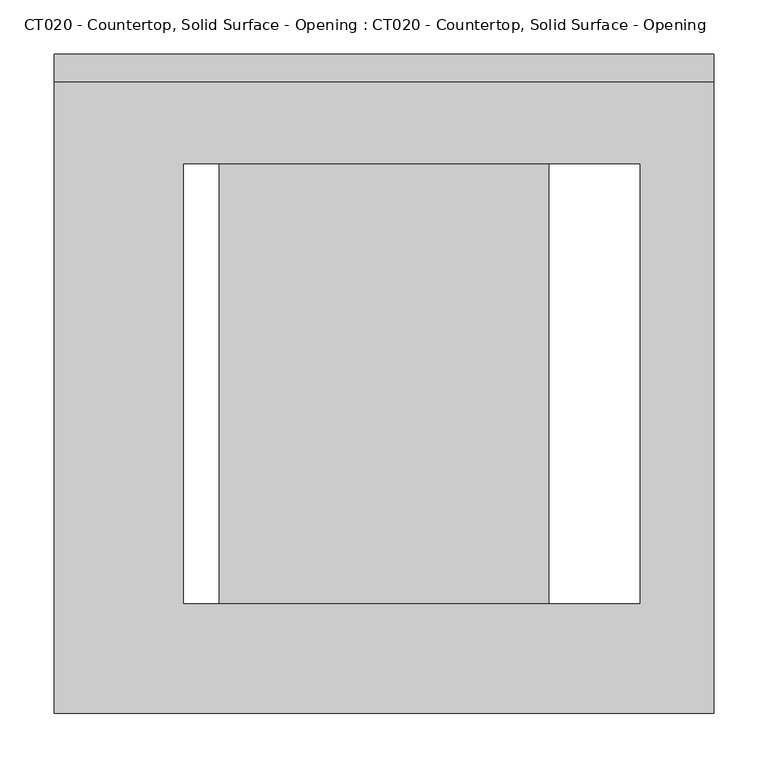
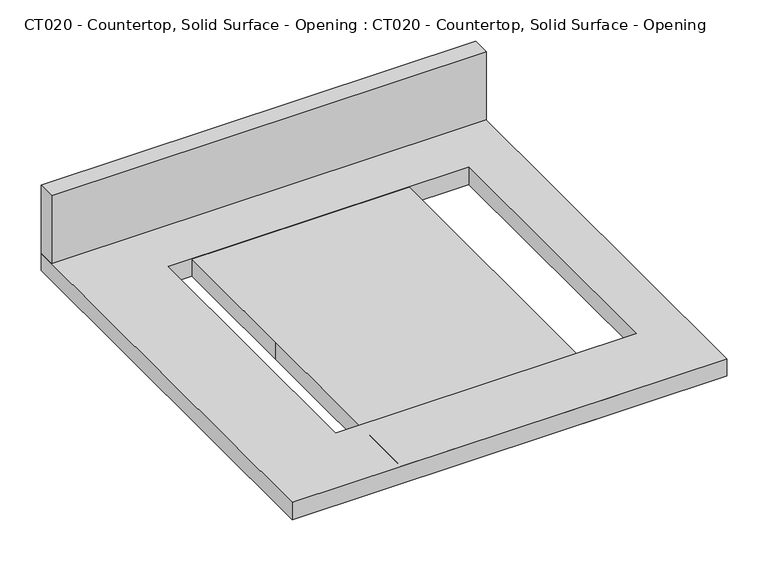
"""IFC4 building model written with IfcOpenShell, lengths in millimetres: proxy geometry, CT020 - Countertop, Solid Surface - Opening : CT020 - Countertop, Solid Surface - Opening."""

from ifc_helpers import new_model, si_unit, frame, origin, origin_with_axes, place, context, project, spatial, polyline, outline, extrude, source, transform, mapped, element, save


def ct020_countertop_solid_surface_opening_ct020_countertop_b7659a89(model_context):
    return source(origin(), model_context, "Body", "SweptSolid", [
        extrude(outline(polyline([(304.8, 304.8), (304.8, -304.8), (-304.8, -304.8), (-304.8, 304.8), (304.8, 304.8)]), holes=[polyline([(236.4002065, 203.2), (-184.9157468, 203.2), (-184.9157468, -203.2), (236.4002065, -203.2), (236.4002065, 203.2)])]), origin_with_axes(), (0.0, 0.0, 1.0), 25.4),
        extrude(outline(polyline([(-304.8, 279.4), (-304.8, 304.8), (304.8, 304.8), (304.8, 279.4), (-304.8, 279.4)])), frame((0.0, 0.0, 25.4), z_axis=(0.0, 0.0, 1.0), x_axis=(1.0, 0.0, 0.0)), (0.0, 0.0, 1.0), 101.6),
        extrude(outline(polyline([(-152.4, 304.8), (152.4, 304.8), (152.4, -304.8), (-152.4, -304.8), (-152.4, 0.0), (-152.4, 304.8)])), origin_with_axes(), (0.0, 0.0, 1.0), 25.4),
    ])


if __name__ == "__main__":
    model = new_model("IFC4")
    model_context = context("Model", 3, world=origin())
    ifc_project = project(units=[si_unit("LENGTHUNIT", "METRE", prefix="MILLI")], contexts=[model_context])
    site = spatial("IfcSite", under=ifc_project)
    building = spatial("IfcBuilding", under=site)
    placement = place(None, origin())
    ct020_countertop_solid_surface_opening_ct020_countertop_shape = ct020_countertop_solid_surface_opening_ct020_countertop_b7659a89(model_context)
    element("IfcBuildingElementProxy", 1, Name="CT020 - Countertop, Solid Surface - Opening : CT020 - Countertop, Solid Surface - Opening", ObjectType="CT020 - Countertop, Solid Surface - Opening : CT020 - Countertop, Solid Surface - Opening", at=placement, inside=building, context=model_context, shape_type="MappedRepresentation", body=[
        mapped(ct020_countertop_solid_surface_opening_ct020_countertop_shape, transform((0.0, 0.0, 0.0), x_axis=(1.0, 0.0, 0.0), y_axis=(0.0, 1.0, 0.0), z_axis=(0.0, 0.0, 1.0))),
    ])
    save(model, "model.ifc")

# Revit data of these elements
# Type "CT020 - Countertop, Solid Surface - Opening : CT020 - Countertop, Solid Surface - Opening"
#   Watts2 = "0"
#   Watts1 = "0"
#   Unit_Issue = "LF"
#   UTIL_6_Misc = "-"
#   UTIL_5_NonMedGas = "-"
#   UTIL_4_MiscGas = "-"
#   UTIL_3_MedGas = "-"
#   UTIL_2_Elec = "-"
#   UTIL_1_WaterDrain = "-"
#   Nomenclature = "Countertop, Solid Surface"
#   NSN = "6530"
#   Location [instance default] = ""
#   JSN = "CT020"
#   Fund_Source_VA = "-"
#   Fund_Source_Navy = "-"
#   Fund_Source_Army = "-"
#   Fund_Source_AF = "-"
#   ELEC_Volts2 = "0"
#   ELEC_Volts1 = "0"
#   ELEC_Phase2 = "0"
#   ELEC_Phase1 = "0"
#   ELEC_HertzSwitch = "0"
#   ELEC_HertzDependent = "0"
#   ELEC_Hertz = "0"
#   ELEC_Amps2 = "0"
#   ELEC_Amps1 = "0"
#   DetailDescription = "High pressure laminate countertop (composition of wood particle core with plastic laminate surface) having a hard smooth surface finish, standard thickness of 1\", and a 4\" butt backsplash/curb. Also referred to as a work surface or work top. Available in a wide choice of colors, patterns, and depths. Used in general purpose areas requiring a basic work surface arrangement with limited heat resistance and poor chemical resistance. Pricing based upon a 24\" depth."
#   CAT_VA = "A"
#   CAT_Navy = "A"
#   CAT_IHS = "-"
#   CAT_Army = "A"
#   CAT_AF = "A"
#   BTUperhour = "0"
#   Weight_IP = 14
#   OpeningLength2 [instance default] = 1' - 6"
#   OpeningLength [instance default] = 2' - 0"
#   OpeningDepth2 [instance default] = 0' - 8"
#   OpeningDepth [instance default] = 0' - 8"
#   DIM_Width_IP = 1' - 0"
#   DIM_Height_IP = 0' - 1"
#   DIM_Depth_IP = 2' - 0"
#   CustomLength2 [instance default] = 1' - 6"
#   CustomLength [instance default] = 6' - 0"
#   Assembly Code = ""
# Element 1 (IfcBuildingElementProxy, "CT020 - Countertop, Solid Surface - Opening : CT020 - Countertop, Solid Surface - Opening")
#   OpeningLength2 = 0' - 9.30709"
#   OpeningLength = 0' - 7.28015"
#   CustomLength = 2' - 0"
#   Materials on its faces: "CounterTopFinish", "EquipSpace"
# Materials
#   "CounterTopFinish": class "Unassigned", colour RGB 139 121 96, transparency 0
#   "EquipSpace": class "Unassigned", colour RGB 221 217 195, transparency 0.5
